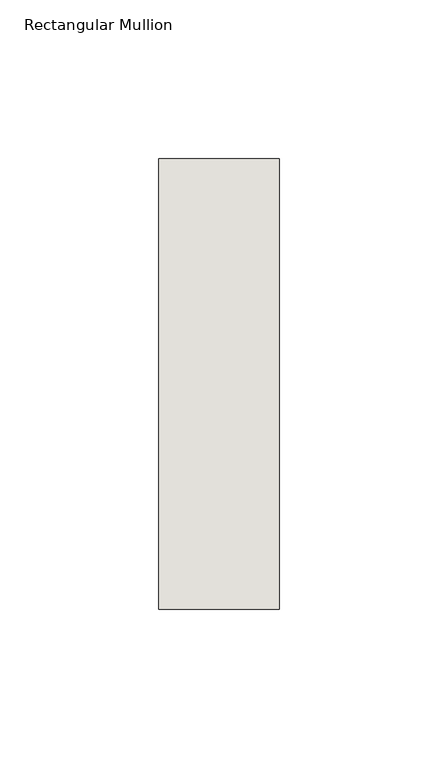
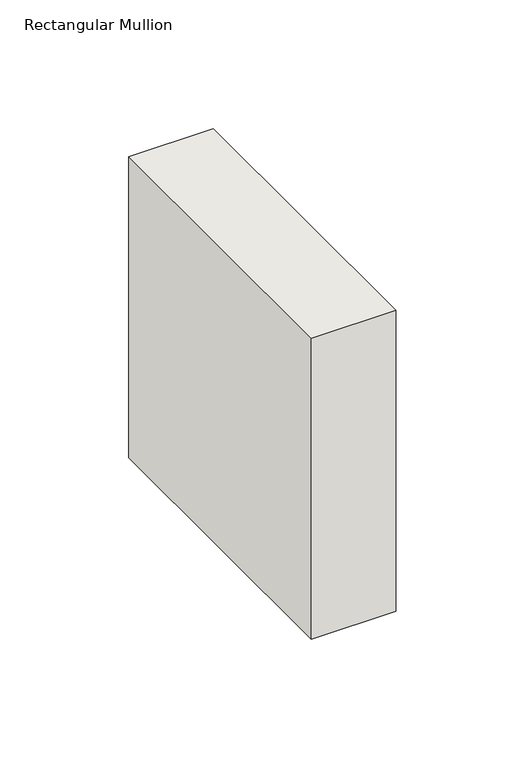
"""IFC4 building model written with IfcOpenShell, lengths in millimetres: wall geometry, Rectangular Mullion : NLRS_21_CWM_hsb-regel 38x142_gen_rsf."""

from ifc_helpers import new_model, si_unit, frame, origin, place, context, project, spatial, polyline, outline, extrude, source, transform, mapped, element, save


def rectangular_mullion_9c2f1ecd(model_context):
    return source(origin(), model_context, "Body", "SweptSolid", [
        extrude(outline(polyline([(-38.0, -71.0), (-38.0, 71.0), (0.0, 71.0), (0.0, -71.0), (-38.0, -71.0)])), frame((0.0, 0.0, -142.9999997), z_axis=(0.0, 0.0, 1.0), x_axis=(1.0, 0.0, 0.0)), (0.0, 0.0, 1.0), 142.9999997),
    ])


if __name__ == "__main__":
    model = new_model("IFC4")
    model_context = context("Model", 3, world=origin())
    ifc_project = project(units=[si_unit("LENGTHUNIT", "METRE", prefix="MILLI")], contexts=[model_context])
    site = spatial("IfcSite", under=ifc_project)
    building = spatial("IfcBuilding", under=site)
    placement = place(None, origin())
    rectangular_mullion_shape = rectangular_mullion_9c2f1ecd(model_context)
    element("IfcWall", 1, ObjectType="Rectangular Mullion : NLRS_21_CWM_hsb-regel 38x142_gen_rsf", at=placement, inside=building, context=model_context, shape_type="MappedRepresentation", body=[
        mapped(rectangular_mullion_shape, transform((0.0, 0.0, 0.0), x_axis=(1.0, 0.0, 0.0), y_axis=(0.0, 1.0, 0.0), z_axis=(0.0, 0.0, 1.0))),
    ])
    save(model, "model.ifc")

# Revit data of these elements
# Type "Rectangular Mullion : NLRS_21_CWM_hsb-regel 38x142_gen_rsf"
#   Type IfcGUID = "07M7mRoiH1CR8m_RSKIwpF"
#   Assembly Code = "21.10"
#   IfcExportAs = "IfcWall"
#   built-in parameter 1007322 = 0.465879 (stored number, unit not read)
#   built-in parameter 1007321 = 0.062336 (stored number, unit not read)
#   built-in parameter 1007320 = 0.062336 (stored number, unit not read)
# Element 1 (IfcWall, "Rectangular Mullion : NLRS_21_CWM_hsb-regel 38x142_gen_rsf")
#   Materials on its faces: "NLRS_i2_hout naaldhout vuren_gen_rsf"
# Materials
#   "NLRS_i2_hout naaldhout vuren_gen_rsf": class "I - Hout", colour RGB 234 199 147, transparency 0, Keynote = "i2", Manufacturer = "Revit Standards Foundation", URL = "www.revitstandards.org", Description = "hout vuren", Cost = 0
